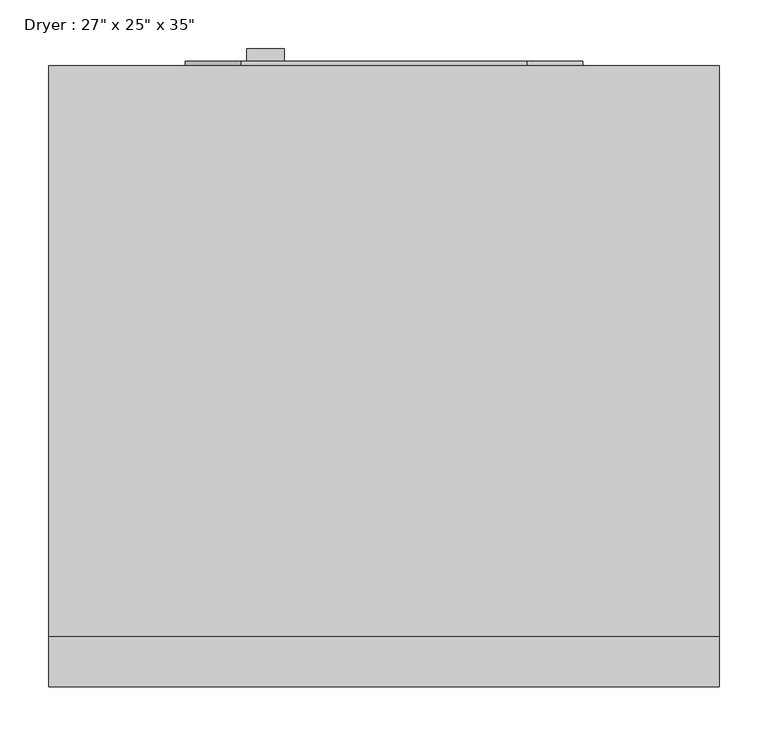
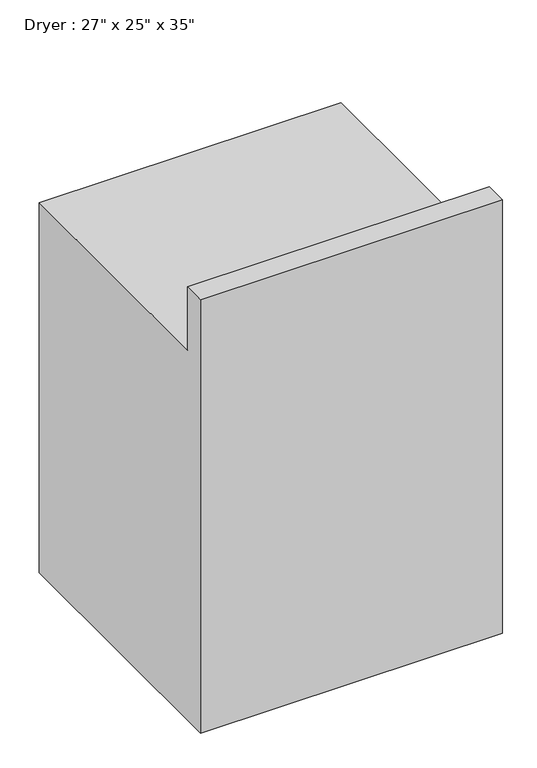
"""IFC4 building model written with IfcOpenShell, lengths in millimetres: proxy geometry."""

from ifc_helpers import new_model, si_unit, point, frame, frame_2d, origin, place, context, project, spatial, polyline, circle_curve, trimmed, segment, composite_curve, outline, extrude, source, transform, mapped, element, save


def proxy_547a9969(model_context):
    return source(origin(), model_context, "Body", "SweptSolid", [
        extrude(outline(polyline([(276.7635206, 20.3014962), (276.7635206, 7.6014962), (238.6635206, 7.6014962), (238.6635206, 20.3014962), (276.7635206, 20.3014962)])), frame((0.0, 0.0, 438.7649313), z_axis=(0.0, 0.0, 1.0), x_axis=(1.0, 0.0, 0.0)), (0.0, 0.0, 1.0), 177.8),
        extrude(outline(composite_curve([segment(polyline([(737.623844, 525.0374563), (737.623844, 232.9374563)]), True, "CONTINUOUS"), segment(trimmed(circle_curve(frame_2d((680.473844, 232.9374563)), 57.15), [point((737.623844, 232.9374563))], [point((680.473844, 175.7874563))], False, "CARTESIAN"), True, "CONTINUOUS"), segment(polyline([(680.473844, 175.7874563), (337.573844, 175.7874563)]), True, "CONTINUOUS"), segment(trimmed(circle_curve(frame_2d((337.573844, 232.9374563)), 57.15), [point((337.573844, 175.7874563))], [point((280.423844, 232.9374563))], False, "CARTESIAN"), True, "CONTINUOUS"), segment(polyline([(280.423844, 232.9374563), (280.423844, 525.0374563)]), True, "CONTINUOUS"), segment(trimmed(circle_curve(frame_2d((337.573844, 525.0374563)), 57.15), [point((280.423844, 525.0374563))], [point((337.573844, 582.1874563))], False, "CARTESIAN"), True, "CONTINUOUS"), segment(polyline([(337.573844, 582.1874563), (680.473844, 582.1874563)]), True, "CONTINUOUS"), segment(trimmed(circle_curve(frame_2d((680.473844, 525.0374563)), 57.15), [point((680.473844, 582.1874563))], [point((737.623844, 525.0374563))], False, "CARTESIAN"), True, "CONTINUOUS")], self_intersect=False)), frame((0.0, 2.8389962, 0.0), z_axis=(0.0, 1.0, 0.0), x_axis=(0.0, 0.0, 1.0)), (0.0, 0.0, 1.0), 4.7625),
        extrude(outline(polyline([(-632.1610038, 0.0), (-632.1610038, 1041.4), (-581.3610038, 1041.4), (-581.3610038, 889.0), (2.8389962, 889.0), (2.8389962, 0.0), (-632.1610038, 0.0)])), frame((36.0874563, 0.0, 0.0), z_axis=(1.0, 0.0, 0.0), x_axis=(0.0, 1.0, 0.0)), (0.0, 0.0, 1.0), 685.8),
    ])


if __name__ == "__main__":
    model = new_model("IFC4")
    model_context = context("Model", 3, world=origin())
    ifc_project = project(units=[si_unit("LENGTHUNIT", "METRE", prefix="MILLI")], contexts=[model_context])
    site = spatial("IfcSite", under=ifc_project)
    building = spatial("IfcBuilding", under=site)
    placement = place(None, origin())
    proxy_shape = proxy_547a9969(model_context)
    element("IfcBuildingElementProxy", 1, Name="Dryer : 27\" x 25\" x 35\"", ObjectType="Dryer : 27\" x 25\" x 35\"", at=placement, inside=building, context=model_context, shape_type="MappedRepresentation", body=[
        mapped(proxy_shape, transform((0.0, 0.0, 0.0), x_axis=(1.0, 0.0, 0.0), y_axis=(0.0, 1.0, 0.0), z_axis=(0.0, 0.0, 1.0))),
    ])
    save(model, "model.ifc")

# Revit data of these elements
# Type "Dryer : 27\" x 25\" x 35\""
#   Label = "D"
#   Assembly Code = "E1090400"
#   Depth = 2' - 1"
#   Height = 2' - 11"
#   Width = 2' - 3"
#   Dryer Material = Metal - Paint Finish - Ivory, Glossy
# Element 1 (IfcBuildingElementProxy, "Dryer : 27\" x 25\" x 35\"")
#   Materials on its faces: "Metal - Paint Finish - Ivory, Glossy"
# Materials
#   "Metal - Paint Finish - Ivory, Glossy": class "Paint", colour RGB 247 247 239, transparency 0
